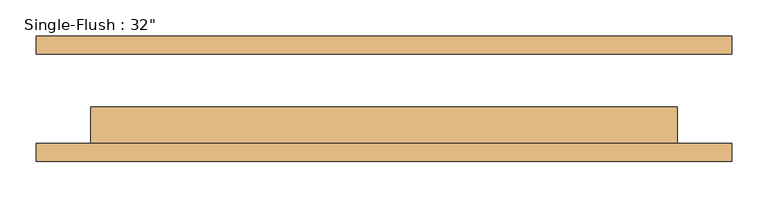
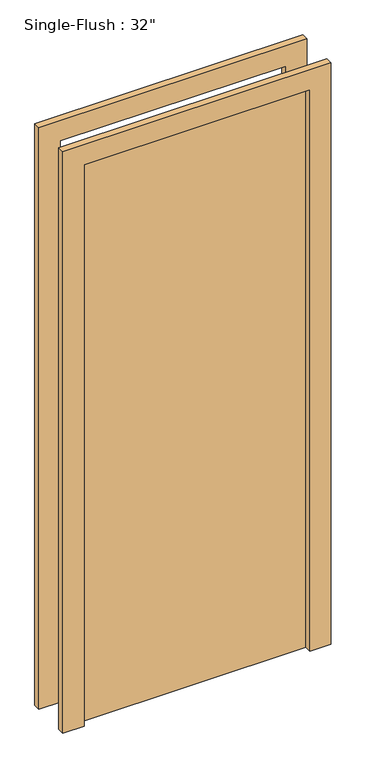
"""IFC4 building model written with IfcOpenShell, lengths in millimetres: door geometry."""

from ifc_helpers import new_model, si_unit, frame, origin, origin_with_axes, place, context, project, spatial, polyline, outline, extrude, source, transform, mapped, element, save


def door_d21431a2(model_context):
    return source(origin(), model_context, "Body", "SweptSolid", [
        extrude(outline(polyline([(2209.8, -482.6), (0.0, -482.6), (0.0, -406.4), (2133.6, -406.4), (2133.6, 406.4), (0.0, 406.4), (0.0, 482.6), (2209.8, 482.6), (2209.8, -482.6)])), frame((0.0, -87.3125, 0.0), z_axis=(0.0, 1.0, 0.0), x_axis=(0.0, 0.0, 1.0)), (0.0, 0.0, 1.0), 25.4),
        extrude(outline(polyline([(2209.8, 482.6), (2209.8, -482.6), (0.0, -482.6), (0.0, -406.4), (2133.6, -406.4), (2133.6, 406.4), (0.0, 406.4), (0.0, 482.6), (2209.8, 482.6)])), frame((0.0, 61.9125, 0.0), z_axis=(0.0, 1.0, 0.0), x_axis=(0.0, 0.0, 1.0)), (0.0, 0.0, 1.0), 25.4),
        extrude(outline(polyline([(406.4, -11.1125), (406.4, -61.9125), (-406.4, -61.9125), (-406.4, -11.1125), (406.4, -11.1125)])), origin_with_axes(), (0.0, 0.0, 1.0), 2133.6),
    ])


if __name__ == "__main__":
    model = new_model("IFC4")
    model_context = context("Model", 3, world=origin())
    ifc_project = project(units=[si_unit("LENGTHUNIT", "METRE", prefix="MILLI")], contexts=[model_context])
    site = spatial("IfcSite", under=ifc_project)
    building = spatial("IfcBuilding", under=site)
    placement = place(None, origin())
    door_shape = door_d21431a2(model_context)
    element("IfcDoor", 1, ObjectType="Single-Flush : 32\"", at=placement, inside=building, context=model_context, shape_type="MappedRepresentation", body=[
        mapped(door_shape, transform((0.0, 0.0, 0.0), x_axis=(1.0, 0.0, 0.0), y_axis=(0.0, 1.0, 0.0), z_axis=(0.0, 0.0, 1.0))),
    ])
    save(model, "model.ifc")

# Revit data of these elements
# Type "Single-Flush : 32\""
#   Type Mark = "57"
#   Construction Type Id = "MDOOR"
#   Assembly Code = "C1020"
#   Analytic Construction = "Metal"
#   Thickness = 0' - 2"
#   Heat Transfer Coefficient (U) = 3.7021 W/(m²·K)
#   Height = 7' - 0"
#   Trim Projection Ext = 0' - 1"
#   Trim Projection Int = 0' - 1"
#   Trim Width = 0' - 3"
#   Width = 2' - 8"
#   Door Material = Door - Panel
#   Frame Material = Door - Frame
#   Visual Light Transmittance = 0
#   Solar Heat Gain Coefficient = 0
#   Function = (empty or 0)
#   Wall Closure = (empty or 0)
# Element 1 (IfcDoor, "Single-Flush : 32\"")
#   Materials on its faces: "Door - Frame", "Door - Panel"
# Materials
#   "Door - Panel": class "Wood", colour RGB 210 159 95, transparency 0
#   "Door - Frame": class "Miscellaneous", colour RGB 118 70 51, transparency 0
